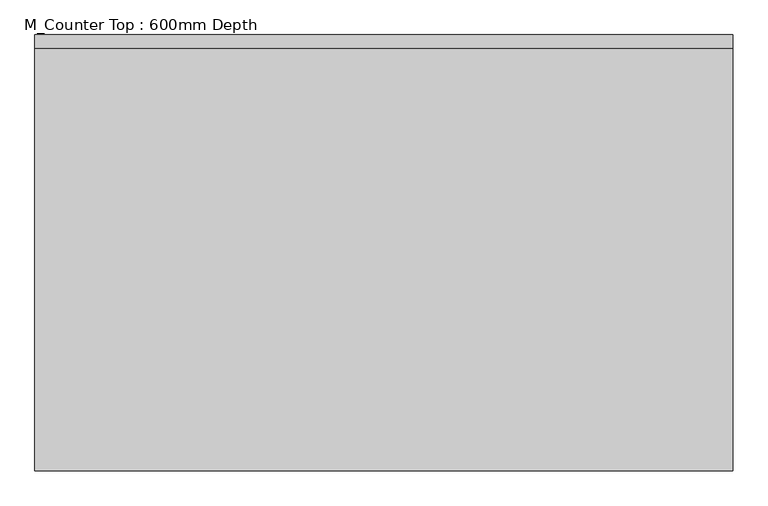
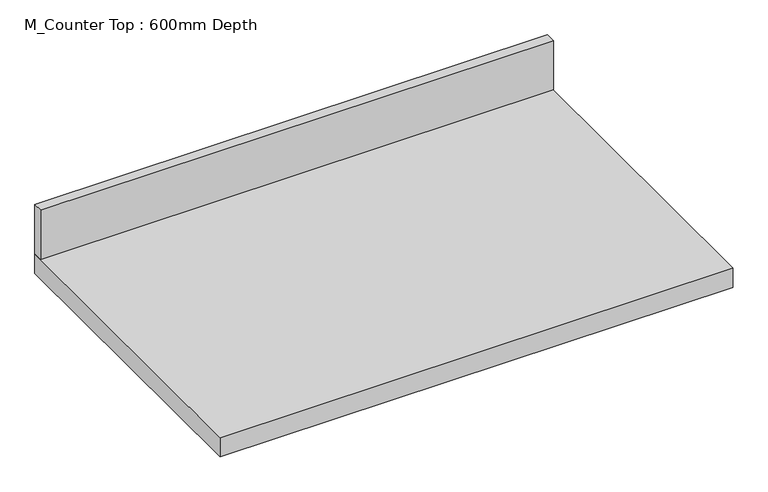
"""IFC4 building model written with IfcOpenShell, lengths in millimetres: furniture geometry, M_Counter Top : 600mm Depth."""

from ifc_helpers import new_model, si_unit, frame, origin, place, context, project, spatial, polyline, outline, extrude, source, transform, mapped, element, save


def m_counter_top_600mm_depth_0fb62e5d(model_context):
    return source(origin(), model_context, "Body", "SweptSolid", [
        extrude(outline(polyline([(-1200.4622951, 0.0), (-200.4622951, 0.0), (-200.4622951, -19.05), (-1200.4622951, -19.05), (-1200.4622951, 0.0)])), frame((0.0, 0.0, 900.0), z_axis=(0.0, 0.0, 1.0), x_axis=(1.0, 0.0, 0.0)), (0.0, 0.0, 1.0), 101.6),
        extrude(outline(polyline([(-200.4622951, 0.0), (-200.4622951, -625.0), (-1200.4622951, -625.0), (-1200.4622951, 0.0), (-200.4622951, 0.0)])), frame((0.0, 0.0, 860.0), z_axis=(0.0, 0.0, 1.0), x_axis=(1.0, 0.0, 0.0)), (0.0, 0.0, 1.0), 40.0),
    ])


if __name__ == "__main__":
    model = new_model("IFC4")
    model_context = context("Model", 3, world=origin())
    ifc_project = project(units=[si_unit("LENGTHUNIT", "METRE", prefix="MILLI")], contexts=[model_context])
    site = spatial("IfcSite", under=ifc_project)
    building = spatial("IfcBuilding", under=site)
    placement = place(None, origin())
    m_counter_top_600mm_depth_shape = m_counter_top_600mm_depth_0fb62e5d(model_context)
    element("IfcFurniture", 1, ObjectType="M_Counter Top : 600mm Depth", at=placement, inside=building, context=model_context, shape_type="MappedRepresentation", body=[
        mapped(m_counter_top_600mm_depth_shape, transform((0.0, 0.0, 0.0), x_axis=(1.0, 0.0, 0.0), y_axis=(0.0, 1.0, 0.0), z_axis=(0.0, 0.0, 1.0))),
    ])
    save(model, "model.ifc")

# Revit data of these elements
# Type "M_Counter Top : 600mm Depth"
#   AccessibilityPerformance = "AccessibilityPerformance"
#   CodePerformance = "CodePerformance"
#   Area = "Area"
#   Color = "Color"
#   Constituents = "Constituents"
#   Features = "Features"
#   Finish = "Finish"
#   Grade = "Grade"
#   Material = "Material"
#   ModelReference = "ModelReference"
#   NominalHeight = "NominalHeight"
#   NominalLength = "NominalLength"
#   NominalWidth = "NominalWidth"
#   ProductionYear = "ProductionYear"
#   Reference = "Reference"
#   Shape = "Shape"
#   Size = "Size"
#   SustainabilityPerformance = "SustainabilityPerformance"
#   WarrantyDescription = "WarrantyDescription"
#   WarrantyDurationLabor = "WarrantyDurationLabor"
#   WarrantyDurationParts = "WarrantyDurationParts"
#   WarrantyGuarantorLabor = "WarrantyGuarantorLabor"
#   WarrantyGuarantorParts = "WarrantyGuarantorParts"
#   ExpectedLife = "ExpectedLife"
#   ReplacementCost = "ReplacementCost"
#   AssetAccountingType = "FIXED"
#   ModelLabel = "ModelLabel"
#   Manufacturer = "Manufacturer"
#   Finish = "Finish"
#   Construction Type = "Construction Type"
#   Counter Thickness = 0.040 m
#   Depth = 0.625 m
#   Height = 0.900 m
#   Length [instance default] = 2.500 m
#   Backsplash Visibility [instance default] = yes
#   Counter Top Material = none
#   Assembly Code = ""
# Element 1 (IfcFurniture, "M_Counter Top : 600mm Depth")
#   Length = 1.000 m
#   Materials on its faces: "Counter Top"
# Materials
#   "Counter Top": class "Wood", colour RGB 226 177 128, transparency 0
